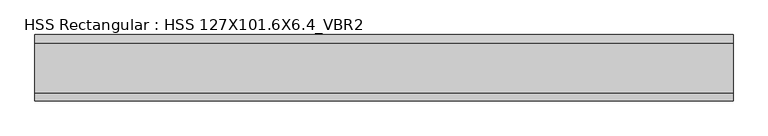
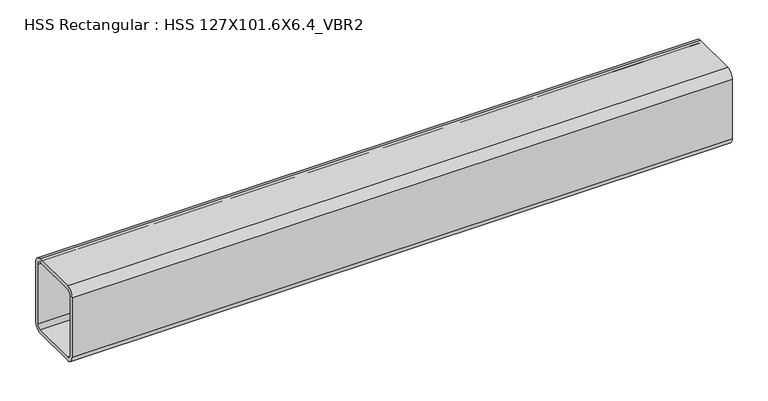
"""IFC4 building model written with IfcOpenShell, lengths in millimetres: member geometry, HSS Rectangular : HSS 127X101.6X6.4_VBR2."""

from ifc_helpers import new_model, si_unit, point, frame, frame_2d, origin, place, context, project, spatial, polyline, circle_curve, trimmed, segment, composite_curve, outline, extrude, source, transform, mapped, element, save


def hss_rectangular_hss_127x101_6x6_4_vbr2_ef6cf57c(model_context):
    return source(origin(), model_context, "Body", "SweptSolid", [
        extrude(outline(composite_curve([segment(polyline([(50.8, 50.8), (50.8, -50.8)]), True, "CONTINUOUS"), segment(trimmed(circle_curve(frame_2d((38.1, -50.8)), 12.7), [point((50.8, -50.8))], [point((38.1, -63.5))], False, "CARTESIAN"), True, "CONTINUOUS"), segment(polyline([(38.1, -63.5), (-38.1, -63.5)]), True, "CONTINUOUS"), segment(trimmed(circle_curve(frame_2d((-38.1, -50.8)), 12.7), [point((-38.1, -63.5))], [point((-50.8, -50.8))], False, "CARTESIAN"), True, "CONTINUOUS"), segment(polyline([(-50.8, -50.8), (-50.8, 50.8)]), True, "CONTINUOUS"), segment(trimmed(circle_curve(frame_2d((-38.1, 50.8)), 12.7), [point((-50.8, 50.8))], [point((-38.1, 63.5))], False, "CARTESIAN"), True, "CONTINUOUS"), segment(polyline([(-38.1, 63.5), (38.1, 63.5)]), True, "CONTINUOUS"), segment(trimmed(circle_curve(frame_2d((38.1, 50.8)), 12.7), [point((38.1, 63.5))], [point((50.8, 50.8))], False, "CARTESIAN"), True, "CONTINUOUS")], self_intersect=False), holes=[composite_curve([segment(trimmed(circle_curve(frame_2d((-38.1, 50.8)), 6.35), [point((-38.1, 57.15))], [point((-44.45, 50.8))], True, "CARTESIAN"), True, "CONTINUOUS"), segment(polyline([(-44.45, 50.8), (-44.45, -50.8)]), True, "CONTINUOUS"), segment(trimmed(circle_curve(frame_2d((-38.1, -50.8)), 6.35), [point((-44.45, -50.8))], [point((-38.1, -57.15))], True, "CARTESIAN"), True, "CONTINUOUS"), segment(polyline([(-38.1, -57.15), (38.1, -57.15)]), True, "CONTINUOUS"), segment(trimmed(circle_curve(frame_2d((38.1, -50.8)), 6.35), [point((38.1, -57.15))], [point((44.45, -50.8))], True, "CARTESIAN"), True, "CONTINUOUS"), segment(polyline([(44.45, -50.8), (44.45, 50.8)]), True, "CONTINUOUS"), segment(trimmed(circle_curve(frame_2d((38.1, 50.8)), 6.35), [point((44.45, 50.8))], [point((38.1, 57.15))], True, "CARTESIAN"), True, "CONTINUOUS"), segment(polyline([(38.1, 57.15), (-38.1, 57.15)]), True, "CONTINUOUS")], self_intersect=False)]), frame((-528.0925542, 0.0, 0.0), z_axis=(1.0, 0.0, 0.0), x_axis=(0.0, 1.0, 0.0)), (0.0, 0.0, 1.0), 1066.2315289),
    ])


if __name__ == "__main__":
    model = new_model("IFC4")
    model_context = context("Model", 3, world=origin())
    ifc_project = project(units=[si_unit("LENGTHUNIT", "METRE", prefix="MILLI")], contexts=[model_context])
    site = spatial("IfcSite", under=ifc_project)
    building = spatial("IfcBuilding", under=site)
    placement = place(None, origin())
    hss_rectangular_hss_127x101_6x6_4_vbr2_shape = hss_rectangular_hss_127x101_6x6_4_vbr2_ef6cf57c(model_context)
    element("IfcMember", 1, ObjectType="HSS Rectangular : HSS 127X101.6X6.4_VBR2", at=placement, inside=building, context=model_context, shape_type="MappedRepresentation", body=[
        mapped(hss_rectangular_hss_127x101_6x6_4_vbr2_shape, transform((0.0, 0.0, 0.0), x_axis=(1.0, 0.0, 0.0), y_axis=(0.0, 1.0, 0.0), z_axis=(0.0, 0.0, 1.0))),
    ])
    save(model, "model.ifc")

# Revit data of these elements
# Type "HSS Rectangular : HSS 127X101.6X6.4_VBR2"
#   Section Name Key = "HSS5X4X1/4"
#   Assembly Code = "B10"
#   Width = 10.16 cm
#   Wall Nominal Thickness = 0.635 cm
#   Wall Design Thickness = 0.5918 cm
#   Torsional Moment of Inertia = 749.217 cm⁴
#   Torsional Modulus = 136.34 cm³
#   Section Area = 24.7741 cm²
#   Plastic Modulus weak axis = 91.2759 cm³
#   Plastic Modulus strong axis = 106.352 cm³
#   Perimeter = 0.435254 m²/m
#   Outer Fillet = 1.27 cm
#   Nominal Weight = 20.7004 kgf/m
#   Moment of Inertia weak axis = 393.755 cm⁴
#   Moment of Inertia strong axis = 557.75 cm⁴
#   Inner Fillet = 0.635 cm
#   Height = 12.7 cm
#   Elastic Modulus weak axis = 77.5108 cm³
#   Elastic Modulus strong axis = 87.6708 cm³
#   Centroid Vertical = 6.35 cm
#   Centroid Horizontal = 5.08 cm
#   Length [instance default] = 1524 mm
#   Structural Material [instance default] = Steel ASTM A500, Grade C, Rectangular and Square
#   Principal Axes Angle = 0
# Element 1 (IfcMember, "HSS Rectangular : HSS 127X101.6X6.4_VBR2")
#   Materials on its faces: "Steel ASTM A500, Grade C, Rectangular and Square"
# Materials
#   "Steel ASTM A500, Grade C, Rectangular and Square": class "Metal", colour RGB 120 120 120, transparency 0, Description = "Carbon steel", Cost = 0
